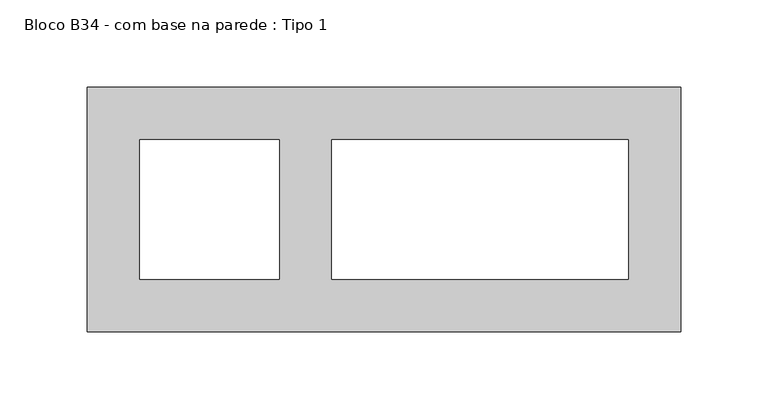
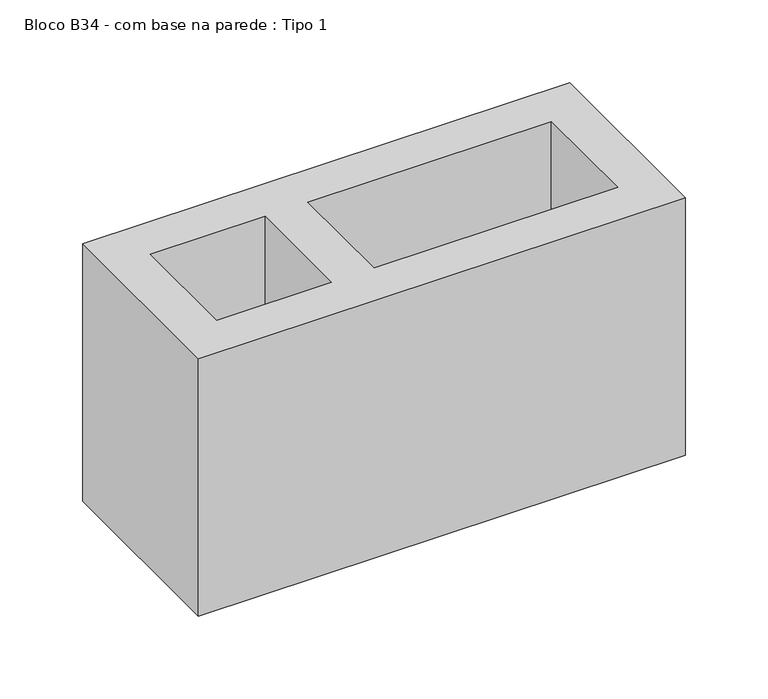
"""IFC4 building model written with IfcOpenShell, lengths in millimetres: proxy geometry, Bloco B34 - com base na parede : Tipo 1."""

from ifc_helpers import new_model, si_unit, origin, origin_with_axes, place, context, project, spatial, polyline, outline, extrude, source, transform, mapped, element, save


def bloco_b34_com_base_na_parede_tipo_1_7f013eb5(model_context):
    return source(origin(), model_context, "Body", "SweptSolid", [
        extrude(outline(polyline([(295.0, -70.0), (-45.0, -70.0), (-45.0, 70.0), (295.0, 70.0), (295.0, -70.0)]), holes=[polyline([(65.0, -40.0), (65.0, 40.0), (-15.0, 40.0), (-15.0, -40.0), (65.0, -40.0)]), polyline([(95.0, -40.0), (265.0, -40.0), (265.0, 40.0), (95.0, 40.0), (95.0, -40.0)])]), origin_with_axes(), (0.0, 0.0, 1.0), 190.0),
    ])


if __name__ == "__main__":
    model = new_model("IFC4")
    model_context = context("Model", 3, world=origin())
    ifc_project = project(units=[si_unit("LENGTHUNIT", "METRE", prefix="MILLI")], contexts=[model_context])
    site = spatial("IfcSite", under=ifc_project)
    building = spatial("IfcBuilding", under=site)
    placement = place(None, origin())
    bloco_b34_com_base_na_parede_tipo_1_shape = bloco_b34_com_base_na_parede_tipo_1_7f013eb5(model_context)
    element("IfcBuildingElementProxy", 1, Name="Bloco B34 - com base na parede : Tipo 1", ObjectType="Bloco B34 - com base na parede : Tipo 1", at=placement, inside=building, context=model_context, shape_type="MappedRepresentation", body=[
        mapped(bloco_b34_com_base_na_parede_tipo_1_shape, transform((0.0, 0.0, 0.0), x_axis=(1.0, 0.0, 0.0), y_axis=(0.0, 1.0, 0.0), z_axis=(0.0, 0.0, 1.0))),
    ])
    save(model, "model.ifc")

# Revit data of these elements
# Type "Bloco B34 - com base na parede : Tipo 1"
#   SINAPI = ""
#   Assembly Code = ""
